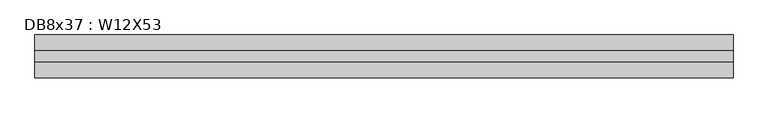
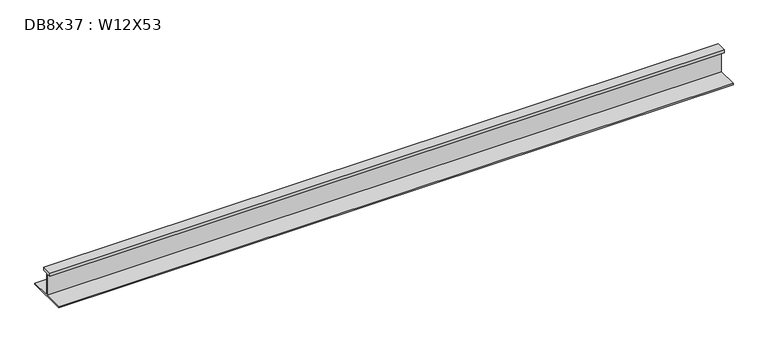
"""IFC4 building model written with IfcOpenShell, lengths in millimetres: beam geometry, DB8x37 : W12X53."""

from ifc_helpers import new_model, si_unit, frame, origin, place, context, project, spatial, polyline, outline, extrude, source, transform, mapped, element, save


def db8x37_w12x53_0f06e810(model_context):
    return source(origin(), model_context, "Body", "SweptSolid", [
        extrude(outline(polyline([(38.1, 145.415), (38.1, 120.015), (2.921, 120.015), (2.921, -48.4505), (152.4, -48.4505), (152.4, -58.1025), (-152.4, -58.1025), (-152.4, -48.4505), (-2.921, -48.4505), (-2.921, 120.015), (-38.1, 120.015), (-38.1, 145.415), (38.1, 145.415)])), frame((-2492.629, 0.0, 0.0), z_axis=(1.0, 0.0, 0.0), x_axis=(0.0, 1.0, 0.0)), (0.0, 0.0, 1.0), 4985.258),
    ])


if __name__ == "__main__":
    model = new_model("IFC4")
    model_context = context("Model", 3, world=origin())
    ifc_project = project(units=[si_unit("LENGTHUNIT", "METRE", prefix="MILLI")], contexts=[model_context])
    site = spatial("IfcSite", under=ifc_project)
    building = spatial("IfcBuilding", under=site)
    placement = place(None, origin())
    db8x37_w12x53_shape = db8x37_w12x53_0f06e810(model_context)
    element("IfcBeam", 1, ObjectType="DB8x37 : W12X53", at=placement, inside=building, context=model_context, shape_type="MappedRepresentation", body=[
        mapped(db8x37_w12x53_shape, transform((0.0, 0.0, 0.0), x_axis=(1.0, 0.0, 0.0), y_axis=(0.0, 1.0, 0.0), z_axis=(0.0, 0.0, 1.0))),
    ])
    save(model, "model.ifc")

# Revit data of these elements
# Type "DB8x37 : W12X53"
#   Assembly Code = "B10"
#   W = 53
#   Length [instance default] = 5' - 0"
#   bf = 0' - 10"
#   d = 1' - 0.1"
#   k = 0' - 1 3/8"
#   k2 = 0' - 0.8"
#   tf = 0' - 0.575"
#   tw = 0' - 0.345"
#   A = 0.108333 SF
#   Structural Material [instance default] = Steel ASTM A992
# Element 1 (IfcBeam, "DB8x37 : W12X53")
#   Materials on its faces: "Steel ASTM A992"
# Materials
#   "Steel ASTM A992": class "Metal", colour RGB 199 199 199, transparency 0, Description = "Structural steel 50ksi", Cost = 0
